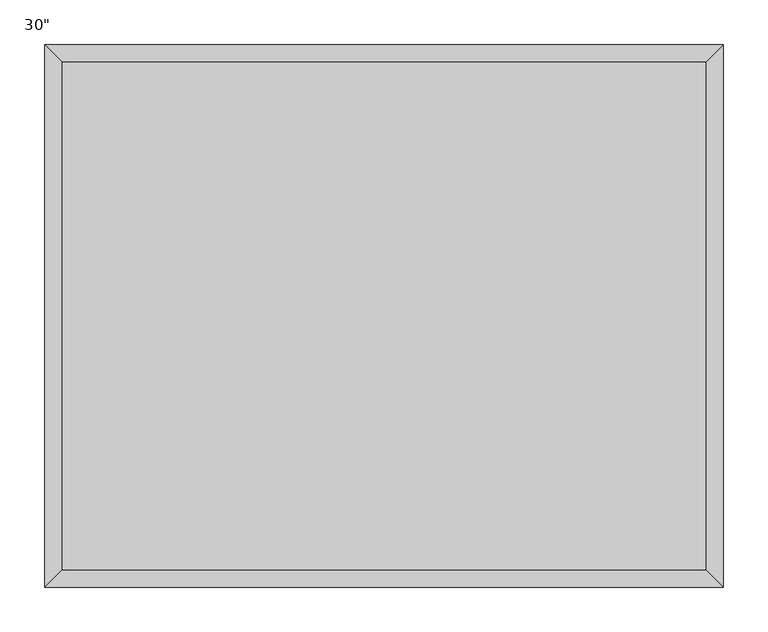
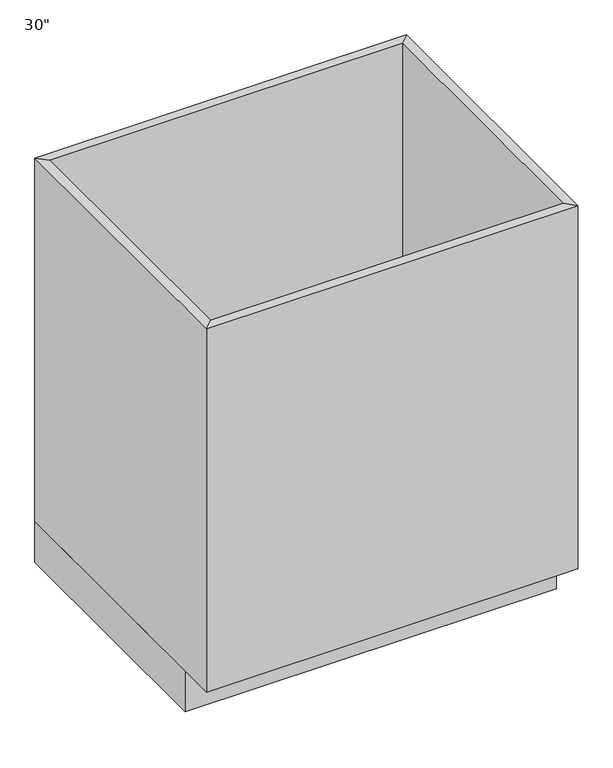
"""IFC4 building model written with IfcOpenShell, lengths in millimetres: furniture geometry."""

import ifcopenshell
import ifcopenshell.guid

model = None  # the IFC model being written
_history = None  # IfcOwnerHistory: only IFC2X3 demands one
_inside = {}  # id of a spatial element -> (the spatial element, [elements in it])
_under = {}  # id of a project, library or spatial element -> (it, [spatial elements below it])
_declared = {}  # id of a project -> (the project, [libraries it declares])
_typed = {}  # id of a type object -> (the type object, [elements of that type])
_made_of = {}  # id of a material, layer set ... -> (it, [elements and type objects made of it])


def new_model(schema):
    """Start an empty IFC model of exactly this schema.

    Asked for "IFC4X3", IfcOpenShell would pick the latest addendum, in which some entities
    have other attributes; the version numbers below select the first issue.
    IFC2X3 requires an IfcOwnerHistory on every rooted entity: one is made here for all.
    """
    global model, _history
    if schema == "IFC4X3":
        model = ifcopenshell.file(schema_version=(4, 3, 0, 0))
    else:
        model = ifcopenshell.file(schema=schema)
    _inside.clear()
    _under.clear()
    _declared.clear()
    _typed.clear()
    _made_of.clear()
    _history = None
    if model.schema == "IFC2X3":
        org = make("IfcOrganization", Name="unknown")
        user = make(
            "IfcPersonAndOrganization",
            ThePerson=make("IfcPerson", FamilyName="unknown"),
            TheOrganization=org,
        )
        app = make(
            "IfcApplication",
            ApplicationDeveloper=org,
            Version="unknown",
            ApplicationFullName="unknown",
            ApplicationIdentifier="unknown",
        )
        _history = make(
            "IfcOwnerHistory",
            OwningUser=user,
            OwningApplication=app,
            ChangeAction="ADDED",
            CreationDate=0,
        )
    return model


def make(cls, **values):
    """One entity of the class cls with the attributes given. An attribute that is None is left unset."""
    return model.create_entity(
        cls, **{name: value for name, value in values.items() if value is not None}
    )


def rooted(cls, **values):
    """An entity with a GlobalId (a new one), such as an element, a storey or a relation."""
    return make(cls, GlobalId=ifcopenshell.guid.new(), OwnerHistory=_history, **values)


def si_unit(unit_type, name, prefix=None):
    """IfcSIUnit, for example si_unit("LENGTHUNIT", "METRE", prefix="MILLI")."""
    return make("IfcSIUnit", UnitType=unit_type, Prefix=prefix, Name=name)


def assignment(units):
    """IfcUnitAssignment: the units of a project."""
    return None if units is None else make("IfcUnitAssignment", Units=units)


def point(xyz):
    """IfcCartesianPoint."""
    return None if xyz is None else make("IfcCartesianPoint", Coordinates=xyz)


def direction(xyz):
    """IfcDirection."""
    return None if xyz is None else make("IfcDirection", DirectionRatios=xyz)


def frame(location, z_axis=None, x_axis=None):
    """IfcAxis2Placement3D, a coordinate frame: its origin and axes. An axis left out is left unset."""
    return make(
        "IfcAxis2Placement3D",
        Location=point(location),
        Axis=direction(z_axis),
        RefDirection=direction(x_axis),
    )


def origin():
    """The frame at (0, 0, 0) with its axes left unset."""
    return frame((0.0, 0.0, 0.0))


def origin_with_axes():
    """The frame at (0, 0, 0) with the z axis (0, 0, 1) and the x axis (1, 0, 0) written out."""
    return frame((0.0, 0.0, 0.0), z_axis=(0.0, 0.0, 1.0), x_axis=(1.0, 0.0, 0.0))


def place(relative_to, where):
    """IfcLocalPlacement: puts the frame where relative to a parent placement (None: the world)."""
    return make(
        "IfcLocalPlacement", PlacementRelTo=relative_to, RelativePlacement=where
    )


def context(
    kind, dimensions, precision=None, world=None, true_north=None, identifier=None
):
    """IfcGeometricRepresentationContext, for example the 3D "Model" context."""
    return make(
        "IfcGeometricRepresentationContext",
        ContextIdentifier=identifier,
        ContextType=kind,
        CoordinateSpaceDimension=dimensions,
        Precision=precision,
        WorldCoordinateSystem=world,
        TrueNorth=true_north,
    )


def project(units=None, contexts=None):
    """IfcProject with its units and contexts."""
    return rooted(
        "IfcProject",
        Name="project",
        RepresentationContexts=contexts,
        UnitsInContext=assignment(units),
    )


def spatial(cls, under=None, at=None, **own):
    """A site, building, storey or space (cls), placed at a placement, below another one or the project."""
    s = rooted(cls, ObjectPlacement=at, **own)
    if under is not None:
        _under.setdefault(under.id(), (under, []))[1].append(s)
    return s


def polyline(points):
    """IfcPolyline through the points."""
    return make("IfcPolyline", Points=[point(p) for p in points])


def outline(outer, holes=None, kind="AREA"):
    """IfcArbitraryClosedProfileDef: a profile drawn as a closed curve; with holes, ...WithVoids."""
    if holes is None:
        return make("IfcArbitraryClosedProfileDef", ProfileType=kind, OuterCurve=outer)
    return make(
        "IfcArbitraryProfileDefWithVoids",
        ProfileType=kind,
        OuterCurve=outer,
        InnerCurves=holes,
    )


def extrude(swept, where, along, depth):
    """IfcExtrudedAreaSolid: the profile swept, set in the frame where, extruded along a direction by depth."""
    return make(
        "IfcExtrudedAreaSolid",
        SweptArea=swept,
        Position=where,
        ExtrudedDirection=direction(along),
        Depth=depth,
    )


def faces_of(points, faces, orient=None, outer=None):
    """IfcFace entities. A face is a list of loops; a loop is a list of indices into points, from 0.

    orient and outer hold one flag for each loop. By default every Orientation is true, the
    first loop of a face is its IfcFaceOuterBound and the others are IfcFaceBound.
    """
    made = []
    for i, loops in enumerate(faces):
        bounds = []
        for j, loop in enumerate(loops):
            is_outer = j == 0 if outer is None else outer[i][j]
            bounds.append(
                make(
                    "IfcFaceOuterBound" if is_outer else "IfcFaceBound",
                    Bound=make("IfcPolyLoop", Polygon=[points[k] for k in loop]),
                    Orientation=True if orient is None else orient[i][j],
                )
            )
        made.append(make("IfcFace", Bounds=bounds))
    return made


def faceted_brep(points, faces, orient=None, outer=None, voids=None):
    """IfcFacetedBrep: a solid bounded by flat faces; with voids (closed shells), ...WithVoids."""
    shared = [point(p) for p in points]
    hull = make("IfcClosedShell", CfsFaces=faces_of(shared, faces, orient, outer))
    if voids is None:
        return make("IfcFacetedBrep", Outer=hull)
    return make(
        "IfcFacetedBrepWithVoids",
        Outer=hull,
        Voids=[
            make(cls, CfsFaces=faces_of(shared, fs, o, b)) for cls, fs, o, b in voids
        ],
    )


def shape(context_of_items, identifier, shape_type, items):
    """IfcShapeRepresentation: the items that make up one representation, for example the "Body"."""
    return make(
        "IfcShapeRepresentation",
        ContextOfItems=context_of_items,
        RepresentationIdentifier=identifier,
        RepresentationType=shape_type,
        Items=items,
    )


def source(mapping_origin, context_of_items, identifier, shape_type, items):
    """IfcRepresentationMap: a shape defined once, which mapped items show again and again."""
    return make(
        "IfcRepresentationMap",
        MappingOrigin=mapping_origin,
        MappedRepresentation=shape(context_of_items, identifier, shape_type, items),
    )


def transform(
    local_origin,
    x_axis=None,
    y_axis=None,
    z_axis=None,
    scale=None,
    scale2=None,
    scale3=None,
    uniform=True,
):
    """IfcCartesianTransformationOperator3D, or its non-uniform kind. x_axis, y_axis, z_axis: its Axis1, 2, 3."""
    if uniform:
        return make(
            "IfcCartesianTransformationOperator3D",
            Axis1=direction(x_axis),
            Axis2=direction(y_axis),
            LocalOrigin=point(local_origin),
            Scale=scale,
            Axis3=direction(z_axis),
        )
    return make(
        "IfcCartesianTransformationOperator3DnonUniform",
        Axis1=direction(x_axis),
        Axis2=direction(y_axis),
        LocalOrigin=point(local_origin),
        Scale=scale,
        Axis3=direction(z_axis),
        Scale2=scale2,
        Scale3=scale3,
    )


def mapped(mapping_source, mapping_target):
    """IfcMappedItem: shows the shape of a source again, moved by a transform."""
    return make(
        "IfcMappedItem", MappingSource=mapping_source, MappingTarget=mapping_target
    )


def made_of(thing, what):
    """Note that an element or type object is made of a material, layer set ...; save() writes the relation."""
    if what is not None:
        _made_of.setdefault(what.id(), (what, []))[1].append(thing)
    return thing


def element(
    cls,
    number,
    at=None,
    inside=None,
    cuts=None,
    type_object=None,
    material=None,
    context=None,
    identifier="Body",
    shape_type=None,
    held_by="IfcProductDefinitionShape",
    body=None,
    shapes=None,
    **own,
):
    """One element of the class cls, such as IfcWall. Its Tag is "e" and its number.

    at: its placement. inside: the storey or other place that contains it. cuts: it is an
    opening in that element (IfcRelVoidsElement). A single representation is given by context,
    identifier, shape_type and body (its items); several are given by shapes. held_by: the class
    of the entity that holds the representations. save() writes the other relations.
    """
    e = rooted(cls, Tag="e%d" % number, ObjectPlacement=at, **own)
    if body is not None:
        shapes = [shape(context, identifier, shape_type, body)]
    if shapes is not None:
        e.Representation = make(held_by, Representations=shapes)
    if inside is not None:
        _inside.setdefault(inside.id(), (inside, []))[1].append(e)
    if cuts is not None:
        rooted(
            "IfcRelVoidsElement", RelatingBuildingElement=cuts, RelatedOpeningElement=e
        )
    if type_object is not None:
        _typed.setdefault(type_object.id(), (type_object, []))[1].append(e)
    return made_of(e, material)


def aggregate(whole, parts):
    """IfcRelAggregates: a whole, such as a stair, and the parts it consists of."""
    return rooted("IfcRelAggregates", RelatingObject=whole, RelatedObjects=parts)


def save(model, path):
    """Write the relations noted so far, then the file.

    IfcRelAggregates (storeys below a building ...), IfcRelContainedInSpatialStructure (elements
    in a storey), IfcRelDefinesByType, IfcRelAssociatesMaterial and IfcRelDeclares: one each for
    every whole, place, type object, material and project.
    """
    for whole, parts in _under.values():
        aggregate(whole, parts)
    for where, things in _inside.values():
        rooted(
            "IfcRelContainedInSpatialStructure",
            RelatedElements=things,
            RelatingStructure=where,
        )
    for kind, things in _typed.values():
        rooted("IfcRelDefinesByType", RelatedObjects=things, RelatingType=kind)
    for what, things in _made_of.values():
        rooted("IfcRelAssociatesMaterial", RelatedObjects=things, RelatingMaterial=what)
    for by, libraries in _declared.values():
        rooted("IfcRelDeclares", RelatingContext=by, RelatedDefinitions=libraries)
    model.write(path)


def furniture_bafe1cba(model_context):
    return source(origin(), model_context, "Body", "SolidModel", [
        extrude(outline(polyline([(380.6877049, -19.05), (380.6877049, -590.55), (-343.2122951, -590.55), (-343.2122951, -19.05), (380.6877049, -19.05)])), frame((0.0, 0.0, 88.9), z_axis=(0.0, 0.0, 1.0), x_axis=(1.0, 0.0, 0.0)), (0.0, 0.0, 1.0), 19.05),
        faceted_brep([(380.6877049, -590.55, 876.3), (380.6877049, -590.55, 88.9), (-343.2122951, -590.55, 88.9), (-343.2122951, -590.55, 876.3), (399.7377049, -609.6, 876.3), (-362.2622951, -609.6, 876.3), (399.7377049, -609.6, 88.9), (-362.2622951, -609.6, 88.9), (-343.2122951, -19.05, 88.9), (-343.2122951, -19.05, 876.3), (-362.2622951, 0.0, 876.3), (-362.2622951, 0.0, 88.9), (380.6877049, -19.05, 88.9), (380.6877049, -19.05, 876.3), (399.7377049, 0.0, 876.3), (399.7377049, 0.0, 88.9)], [[[0, 1, 2, 3]], [[4, 0, 3, 5]], [[6, 4, 5, 7]], [[1, 6, 7, 2]], [[3, 2, 8, 9]], [[5, 3, 9, 10]], [[7, 5, 10, 11]], [[2, 7, 11, 8]], [[9, 8, 12, 13]], [[10, 9, 13, 14]], [[11, 10, 14, 15]], [[8, 11, 15, 12]], [[13, 12, 1, 0]], [[14, 13, 0, 4]], [[15, 14, 4, 6]], [[12, 15, 6, 1]]]),
        extrude(outline(polyline([(399.7377049, 0.0), (399.7377049, -533.4), (-362.2622951, -533.4), (-362.2622951, 0.0), (399.7377049, 0.0)])), origin_with_axes(), (0.0, 0.0, 1.0), 88.9),
    ])


if __name__ == "__main__":
    model = new_model("IFC4")
    model_context = context("Model", 3, world=origin())
    ifc_project = project(units=[si_unit("LENGTHUNIT", "METRE", prefix="MILLI")], contexts=[model_context])
    site = spatial("IfcSite", under=ifc_project)
    building = spatial("IfcBuilding", under=site)
    placement = place(None, origin())
    furniture_shape = furniture_bafe1cba(model_context)
    element("IfcFurniture", 1, ObjectType="Base Cabinet-Double Door & 1 Drawer : 30\"", at=placement, inside=building, context=model_context, shape_type="MappedRepresentation", body=[
        mapped(furniture_shape, transform((0.0, 0.0, 0.0), x_axis=(1.0, 0.0, 0.0), y_axis=(0.0, 1.0, 0.0), z_axis=(0.0, 0.0, 1.0))),
    ])
    save(model, "model.ifc")

# Revit data of these elements
# Type "Base Cabinet-Double Door & 1 Drawer : 30\""
#   Finish = "Cabinetry"
#   Depth = 2' - 0"
#   Height = 2' - 10 1/2"
#   Toe Depth = 0' - 3"
#   Toe Height = 0' - 3 1/2"
#   Width = 2' - 6"
# Element 1 (IfcFurniture, "Base Cabinet-Double Door & 1 Drawer : 30\"")
#   Materials on its faces: "Cabinet"
# Materials
#   "Cabinet": class "Wood", colour RGB 189 170 130, transparency 0, Cost = 0
